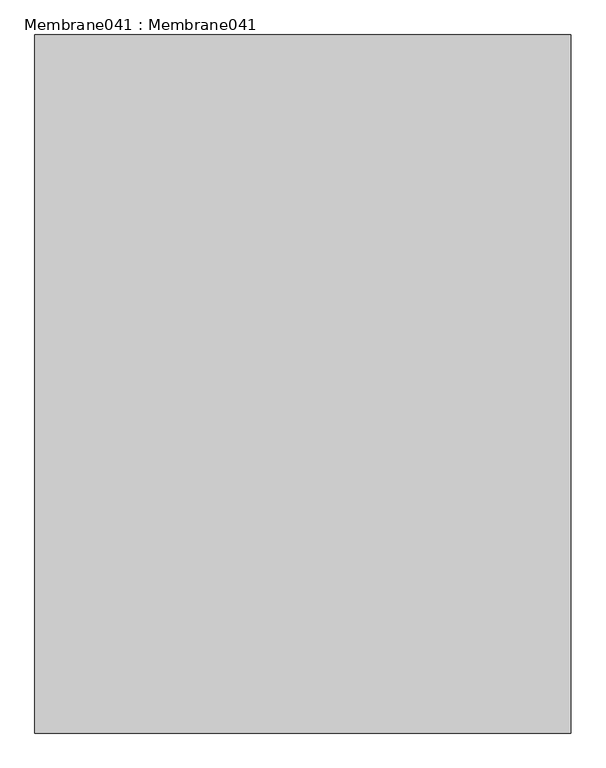
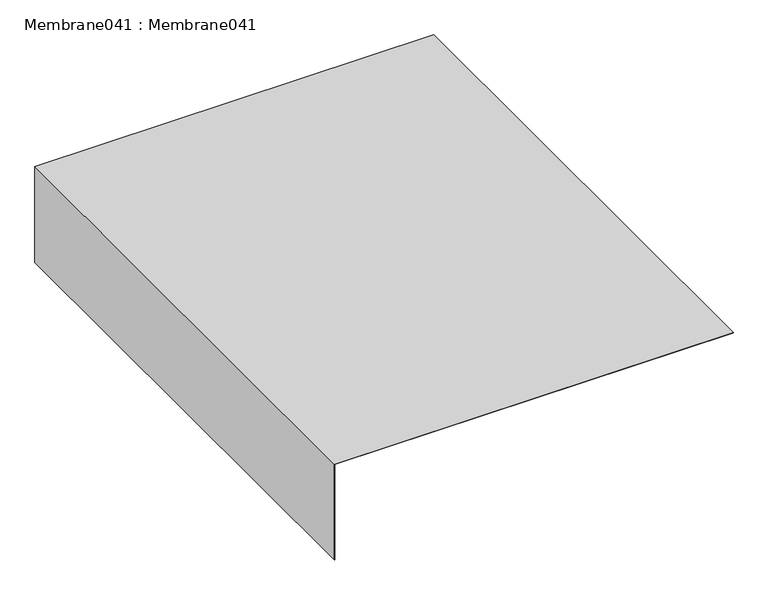
"""IFC4 building model written with IfcOpenShell, lengths in millimetres: proxy geometry, Membrane041 : Membrane041."""

import ifcopenshell
import ifcopenshell.guid

model = None  # the IFC model being written
_history = None  # IfcOwnerHistory: only IFC2X3 demands one
_inside = {}  # id of a spatial element -> (the spatial element, [elements in it])
_under = {}  # id of a project, library or spatial element -> (it, [spatial elements below it])
_declared = {}  # id of a project -> (the project, [libraries it declares])
_typed = {}  # id of a type object -> (the type object, [elements of that type])
_made_of = {}  # id of a material, layer set ... -> (it, [elements and type objects made of it])


def new_model(schema):
    """Start an empty IFC model of exactly this schema.

    Asked for "IFC4X3", IfcOpenShell would pick the latest addendum, in which some entities
    have other attributes; the version numbers below select the first issue.
    IFC2X3 requires an IfcOwnerHistory on every rooted entity: one is made here for all.
    """
    global model, _history
    if schema == "IFC4X3":
        model = ifcopenshell.file(schema_version=(4, 3, 0, 0))
    else:
        model = ifcopenshell.file(schema=schema)
    _inside.clear()
    _under.clear()
    _declared.clear()
    _typed.clear()
    _made_of.clear()
    _history = None
    if model.schema == "IFC2X3":
        org = make("IfcOrganization", Name="unknown")
        user = make(
            "IfcPersonAndOrganization",
            ThePerson=make("IfcPerson", FamilyName="unknown"),
            TheOrganization=org,
        )
        app = make(
            "IfcApplication",
            ApplicationDeveloper=org,
            Version="unknown",
            ApplicationFullName="unknown",
            ApplicationIdentifier="unknown",
        )
        _history = make(
            "IfcOwnerHistory",
            OwningUser=user,
            OwningApplication=app,
            ChangeAction="ADDED",
            CreationDate=0,
        )
    return model


def make(cls, **values):
    """One entity of the class cls with the attributes given. An attribute that is None is left unset."""
    return model.create_entity(
        cls, **{name: value for name, value in values.items() if value is not None}
    )


def rooted(cls, **values):
    """An entity with a GlobalId (a new one), such as an element, a storey or a relation."""
    return make(cls, GlobalId=ifcopenshell.guid.new(), OwnerHistory=_history, **values)


def si_unit(unit_type, name, prefix=None):
    """IfcSIUnit, for example si_unit("LENGTHUNIT", "METRE", prefix="MILLI")."""
    return make("IfcSIUnit", UnitType=unit_type, Prefix=prefix, Name=name)


def assignment(units):
    """IfcUnitAssignment: the units of a project."""
    return None if units is None else make("IfcUnitAssignment", Units=units)


def point(xyz):
    """IfcCartesianPoint."""
    return None if xyz is None else make("IfcCartesianPoint", Coordinates=xyz)


def direction(xyz):
    """IfcDirection."""
    return None if xyz is None else make("IfcDirection", DirectionRatios=xyz)


def frame(location, z_axis=None, x_axis=None):
    """IfcAxis2Placement3D, a coordinate frame: its origin and axes. An axis left out is left unset."""
    return make(
        "IfcAxis2Placement3D",
        Location=point(location),
        Axis=direction(z_axis),
        RefDirection=direction(x_axis),
    )


def origin():
    """The frame at (0, 0, 0) with its axes left unset."""
    return frame((0.0, 0.0, 0.0))


def place(relative_to, where):
    """IfcLocalPlacement: puts the frame where relative to a parent placement (None: the world)."""
    return make(
        "IfcLocalPlacement", PlacementRelTo=relative_to, RelativePlacement=where
    )


def context(
    kind, dimensions, precision=None, world=None, true_north=None, identifier=None
):
    """IfcGeometricRepresentationContext, for example the 3D "Model" context."""
    return make(
        "IfcGeometricRepresentationContext",
        ContextIdentifier=identifier,
        ContextType=kind,
        CoordinateSpaceDimension=dimensions,
        Precision=precision,
        WorldCoordinateSystem=world,
        TrueNorth=true_north,
    )


def project(units=None, contexts=None):
    """IfcProject with its units and contexts."""
    return rooted(
        "IfcProject",
        Name="project",
        RepresentationContexts=contexts,
        UnitsInContext=assignment(units),
    )


def spatial(cls, under=None, at=None, **own):
    """A site, building, storey or space (cls), placed at a placement, below another one or the project."""
    s = rooted(cls, ObjectPlacement=at, **own)
    if under is not None:
        _under.setdefault(under.id(), (under, []))[1].append(s)
    return s


def polyline(points):
    """IfcPolyline through the points."""
    return make("IfcPolyline", Points=[point(p) for p in points])


def outline(outer, holes=None, kind="AREA"):
    """IfcArbitraryClosedProfileDef: a profile drawn as a closed curve; with holes, ...WithVoids."""
    if holes is None:
        return make("IfcArbitraryClosedProfileDef", ProfileType=kind, OuterCurve=outer)
    return make(
        "IfcArbitraryProfileDefWithVoids",
        ProfileType=kind,
        OuterCurve=outer,
        InnerCurves=holes,
    )


def extrude(swept, where, along, depth):
    """IfcExtrudedAreaSolid: the profile swept, set in the frame where, extruded along a direction by depth."""
    return make(
        "IfcExtrudedAreaSolid",
        SweptArea=swept,
        Position=where,
        ExtrudedDirection=direction(along),
        Depth=depth,
    )


def shape(context_of_items, identifier, shape_type, items):
    """IfcShapeRepresentation: the items that make up one representation, for example the "Body"."""
    return make(
        "IfcShapeRepresentation",
        ContextOfItems=context_of_items,
        RepresentationIdentifier=identifier,
        RepresentationType=shape_type,
        Items=items,
    )


def source(mapping_origin, context_of_items, identifier, shape_type, items):
    """IfcRepresentationMap: a shape defined once, which mapped items show again and again."""
    return make(
        "IfcRepresentationMap",
        MappingOrigin=mapping_origin,
        MappedRepresentation=shape(context_of_items, identifier, shape_type, items),
    )


def transform(
    local_origin,
    x_axis=None,
    y_axis=None,
    z_axis=None,
    scale=None,
    scale2=None,
    scale3=None,
    uniform=True,
):
    """IfcCartesianTransformationOperator3D, or its non-uniform kind. x_axis, y_axis, z_axis: its Axis1, 2, 3."""
    if uniform:
        return make(
            "IfcCartesianTransformationOperator3D",
            Axis1=direction(x_axis),
            Axis2=direction(y_axis),
            LocalOrigin=point(local_origin),
            Scale=scale,
            Axis3=direction(z_axis),
        )
    return make(
        "IfcCartesianTransformationOperator3DnonUniform",
        Axis1=direction(x_axis),
        Axis2=direction(y_axis),
        LocalOrigin=point(local_origin),
        Scale=scale,
        Axis3=direction(z_axis),
        Scale2=scale2,
        Scale3=scale3,
    )


def mapped(mapping_source, mapping_target):
    """IfcMappedItem: shows the shape of a source again, moved by a transform."""
    return make(
        "IfcMappedItem", MappingSource=mapping_source, MappingTarget=mapping_target
    )


def made_of(thing, what):
    """Note that an element or type object is made of a material, layer set ...; save() writes the relation."""
    if what is not None:
        _made_of.setdefault(what.id(), (what, []))[1].append(thing)
    return thing


def element(
    cls,
    number,
    at=None,
    inside=None,
    cuts=None,
    type_object=None,
    material=None,
    context=None,
    identifier="Body",
    shape_type=None,
    held_by="IfcProductDefinitionShape",
    body=None,
    shapes=None,
    **own,
):
    """One element of the class cls, such as IfcWall. Its Tag is "e" and its number.

    at: its placement. inside: the storey or other place that contains it. cuts: it is an
    opening in that element (IfcRelVoidsElement). A single representation is given by context,
    identifier, shape_type and body (its items); several are given by shapes. held_by: the class
    of the entity that holds the representations. save() writes the other relations.
    """
    e = rooted(cls, Tag="e%d" % number, ObjectPlacement=at, **own)
    if body is not None:
        shapes = [shape(context, identifier, shape_type, body)]
    if shapes is not None:
        e.Representation = make(held_by, Representations=shapes)
    if inside is not None:
        _inside.setdefault(inside.id(), (inside, []))[1].append(e)
    if cuts is not None:
        rooted(
            "IfcRelVoidsElement", RelatingBuildingElement=cuts, RelatedOpeningElement=e
        )
    if type_object is not None:
        _typed.setdefault(type_object.id(), (type_object, []))[1].append(e)
    return made_of(e, material)


def aggregate(whole, parts):
    """IfcRelAggregates: a whole, such as a stair, and the parts it consists of."""
    return rooted("IfcRelAggregates", RelatingObject=whole, RelatedObjects=parts)


def save(model, path):
    """Write the relations noted so far, then the file.

    IfcRelAggregates (storeys below a building ...), IfcRelContainedInSpatialStructure (elements
    in a storey), IfcRelDefinesByType, IfcRelAssociatesMaterial and IfcRelDeclares: one each for
    every whole, place, type object, material and project.
    """
    for whole, parts in _under.values():
        aggregate(whole, parts)
    for where, things in _inside.values():
        rooted(
            "IfcRelContainedInSpatialStructure",
            RelatedElements=things,
            RelatingStructure=where,
        )
    for kind, things in _typed.values():
        rooted("IfcRelDefinesByType", RelatedObjects=things, RelatingType=kind)
    for what, things in _made_of.values():
        rooted("IfcRelAssociatesMaterial", RelatedObjects=things, RelatingMaterial=what)
    for by, libraries in _declared.values():
        rooted("IfcRelDeclares", RelatingContext=by, RelatedDefinitions=libraries)
    model.write(path)


def membrane041_membrane041_8a17b6ef(model_context):
    return source(origin(), model_context, "Body", "SweptSolid", [
        extrude(outline(polyline([(43443.8828125, -4953.168457), (43443.8828125, -6489.7270508), (43053.9921875, -6489.7270508), (43053.9921875, -6487.7270508), (43441.8828125, -6487.7270508), (43441.8828125, -4953.168457), (43443.8828125, -4953.168457)])), frame((0.0, 7982.1531721, 0.0), z_axis=(0.0, 1.0, 0.0), x_axis=(0.0, 0.0, 1.0)), (0.0, 0.0, 1.0), 2000.0),
    ])


if __name__ == "__main__":
    model = new_model("IFC4")
    model_context = context("Model", 3, world=origin())
    ifc_project = project(units=[si_unit("LENGTHUNIT", "METRE", prefix="MILLI")], contexts=[model_context])
    site = spatial("IfcSite", under=ifc_project)
    building = spatial("IfcBuilding", under=site)
    placement = place(None, origin())
    membrane041_membrane041_shape = membrane041_membrane041_8a17b6ef(model_context)
    element("IfcBuildingElementProxy", 1, Name="Membrane041 : Membrane041", ObjectType="Membrane041 : Membrane041", at=placement, inside=building, context=model_context, shape_type="MappedRepresentation", body=[
        mapped(membrane041_membrane041_shape, transform((0.0, 0.0, 0.0), x_axis=(1.0, 0.0, 0.0), y_axis=(0.0, 1.0, 0.0), z_axis=(0.0, 0.0, 1.0))),
    ])
    save(model, "model.ifc")

# Revit data of these elements
# Type "Membrane041 : Membrane041"
#   NameOverride = "Membrane041"
# Element 1 (IfcBuildingElementProxy, "Membrane041 : Membrane041")
#   Materials on its faces: "ASPHALT SATURATED ORGANIC FELT @ ROOF"
# Materials
#   "ASPHALT SATURATED ORGANIC FELT @ ROOF": class "Unassigned", colour RGB 85 170 127, transparency 0
